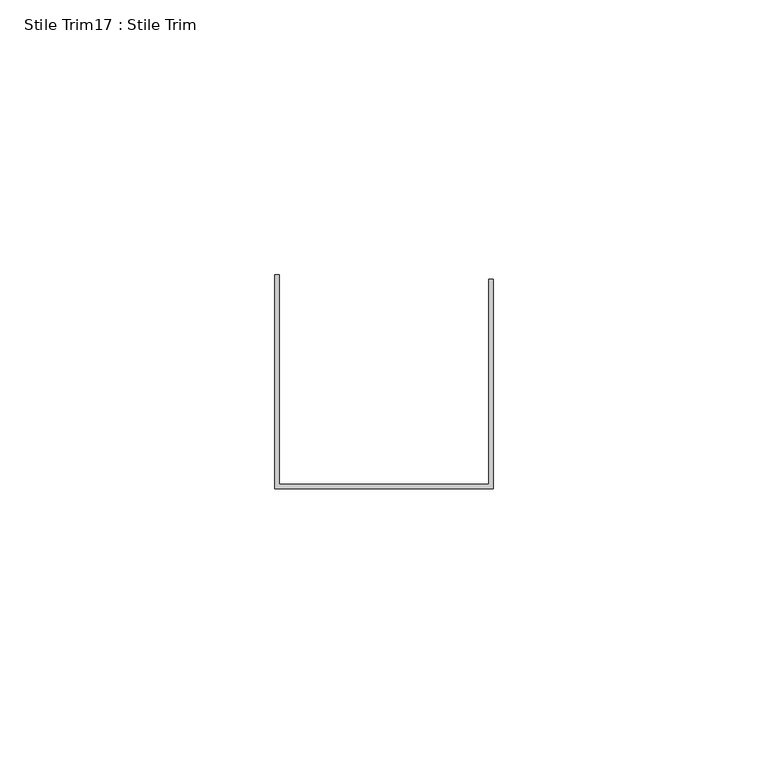
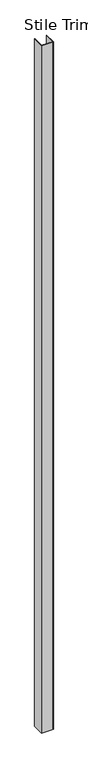
"""IFC4 building model written with IfcOpenShell, lengths in millimetres: proxy geometry, Stile Trim17 : Stile Trim."""

from ifc_helpers import new_model, si_unit, frame, origin, place, context, project, spatial, polyline, outline, extrude, source, transform, mapped, element, save


def stile_trim17_stile_trim_8294cd2f(model_context):
    return source(origin(), model_context, "Body", "SweptSolid", [
        extrude(outline(polyline([(587327.0060739, -536420.7663841), (587327.0060739, -536381.8789841), (587327.7934739, -536381.8789841), (587327.7934739, -536419.9789841), (587365.8934739, -536419.9789841), (587365.8934739, -536382.6663841), (587366.6808739, -536382.6663841), (587366.6808739, -536420.7663841), (587327.0060739, -536420.7663841)])), frame((0.0, 0.0, 12.7), z_axis=(0.0, 0.0, 1.0), x_axis=(1.0, 0.0, 0.0)), (0.0, 0.0, 1.0), 2425.7),
    ])


if __name__ == "__main__":
    model = new_model("IFC4")
    model_context = context("Model", 3, world=origin())
    ifc_project = project(units=[si_unit("LENGTHUNIT", "METRE", prefix="MILLI")], contexts=[model_context])
    site = spatial("IfcSite", under=ifc_project)
    building = spatial("IfcBuilding", under=site)
    placement = place(None, origin())
    stile_trim17_stile_trim_shape = stile_trim17_stile_trim_8294cd2f(model_context)
    element("IfcBuildingElementProxy", 1, Name="Stile Trim17 : Stile Trim", ObjectType="Stile Trim17 : Stile Trim", at=placement, inside=building, context=model_context, shape_type="MappedRepresentation", body=[
        mapped(stile_trim17_stile_trim_shape, transform((0.0, 0.0, 0.0), x_axis=(1.0, 0.0, 0.0), y_axis=(0.0, 1.0, 0.0), z_axis=(0.0, 0.0, 1.0))),
    ])
    save(model, "model.ifc")

# Revit data of these elements
# Element 1 (IfcBuildingElementProxy, "Stile Trim17 : Stile Trim")
#   Materials on its faces: "EDGE TRIM BY MTL PANEL MFR."
# Materials
#   "EDGE TRIM BY MTL PANEL MFR.": class "Generic", colour RGB 239 242 240, transparency 0, Cost = 0
